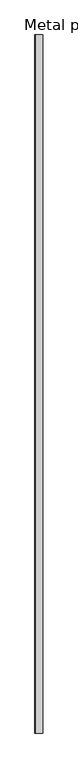
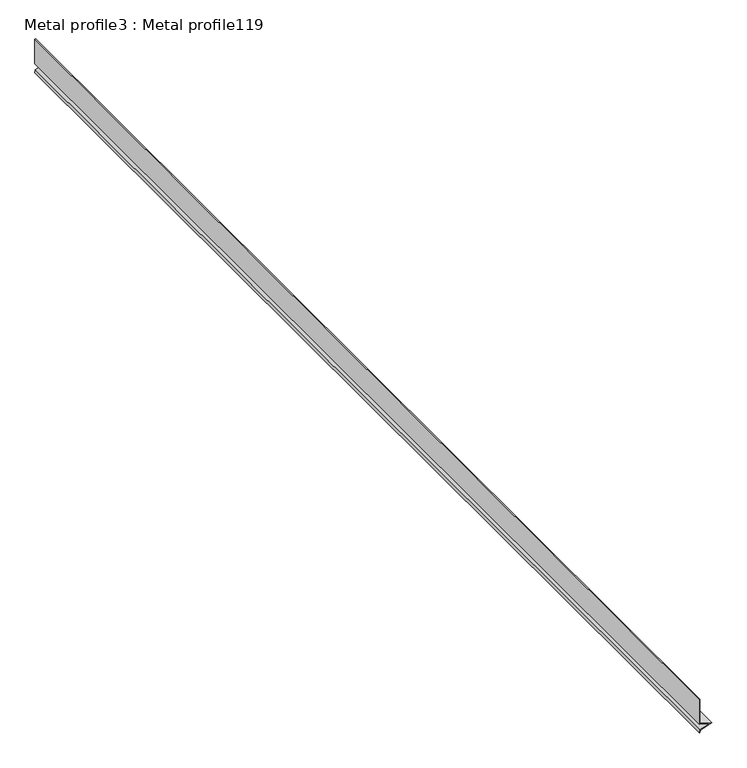
"""IFC4 building model written with IfcOpenShell, lengths in millimetres: proxy geometry, Metal profile3 : Metal profile119."""

from ifc_helpers import new_model, si_unit, frame, origin, place, context, project, spatial, polyline, outline, extrude, source, transform, mapped, element, save


def metal_profile3_metal_profile119_f4195073(model_context):
    return source(origin(), model_context, "Body", "SweptSolid", [
        extrude(outline(polyline([(40157.1419344, 16504.9697926), (40157.1419344, 16503.6997926), (40112.1516908, 16503.6997926), (40106.3419344, 16521.7745903), (40100.8417764, 16504.6629877), (40095.727026, 16503.6997926), (40095.4919945, 16504.9478551), (40099.8639862, 16505.7711761), (40106.3419328, 16525.9247876), (40113.0774701, 16504.9697926), (40157.1419344, 16504.9697926)])), frame((0.0, -1052.8906567, 0.0), z_axis=(0.0, 1.0, 0.0), x_axis=(0.0, 0.0, 1.0)), (0.0, 0.0, 1.0), 1999.85),
    ])


if __name__ == "__main__":
    model = new_model("IFC4")
    model_context = context("Model", 3, world=origin())
    ifc_project = project(units=[si_unit("LENGTHUNIT", "METRE", prefix="MILLI")], contexts=[model_context])
    site = spatial("IfcSite", under=ifc_project)
    building = spatial("IfcBuilding", under=site)
    placement = place(None, origin())
    metal_profile3_metal_profile119_shape = metal_profile3_metal_profile119_f4195073(model_context)
    element("IfcBuildingElementProxy", 1, Name="Metal profile3 : Metal profile119", ObjectType="Metal profile3 : Metal profile119", at=placement, inside=building, context=model_context, shape_type="MappedRepresentation", body=[
        mapped(metal_profile3_metal_profile119_shape, transform((0.0, 0.0, 0.0), x_axis=(1.0, 0.0, 0.0), y_axis=(0.0, 1.0, 0.0), z_axis=(0.0, 0.0, 1.0))),
    ])
    save(model, "model.ifc")

# Revit data of these elements
# Type "Metal profile3 : Metal profile119"
#   NameOverride = "Metal profile119"
# Element 1 (IfcBuildingElementProxy, "Metal profile3 : Metal profile119")
#   Materials on its faces: "16 GA. COPPER WEEP SCREED W/ MIN 3 1/2\" ATTACHMENT FLANGE - LAP UNDERLAYMENT OVER WEED SCREED"
# Materials
#   "16 GA. COPPER WEEP SCREED W/ MIN 3 1/2\" ATTACHMENT FLANGE - LAP UNDERLAYMENT OVER WEED SCREED": class "Unassigned", colour RGB 251 232 155, transparency 0, Cost = 0
